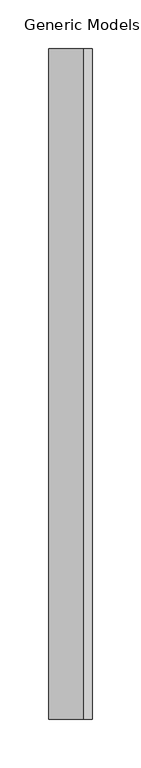
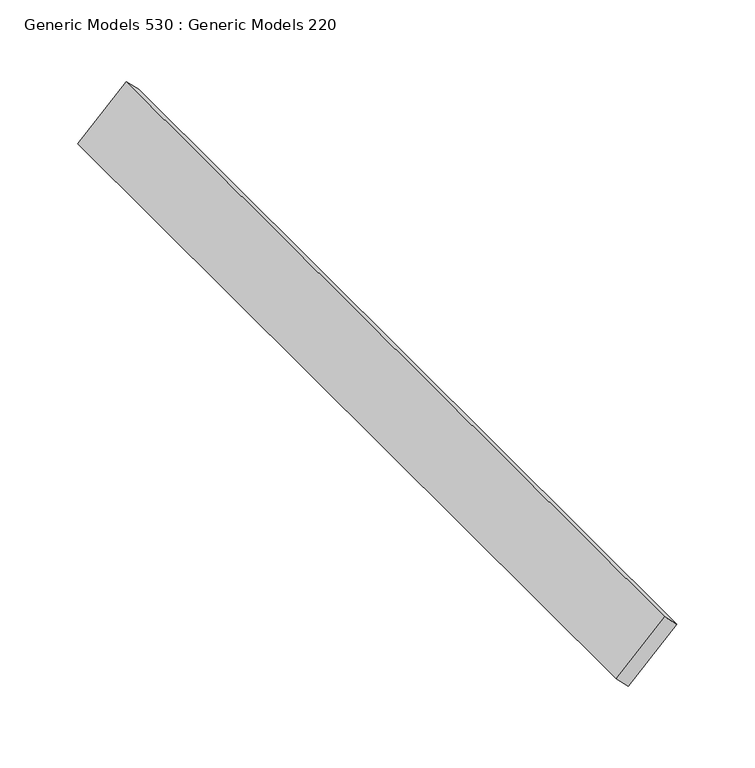
"""IFC4 building model written with IfcOpenShell, lengths in millimetres: proxy geometry, Generic Models 530 : Generic Models 220."""

from ifc_helpers import new_model, si_unit, frame, origin, place, context, project, spatial, polyline, outline, extrude, source, transform, mapped, element, save


def generic_models_530_generic_models_220_b77ca90a(model_context):
    return source(origin(), model_context, "Body", "SweptSolid", [
        extrude(outline(polyline([(0.0, -12.7000001), (0.0, 0.0), (690.8142348, 0.0), (690.8142348, -12.7000001), (0.0, -12.7000001)])), frame((7841.3059863, 4539.4872686, 125319.1399101), z_axis=(0.7071067811868034, 0.0, 0.7071067811862918), x_axis=(0.0, -1.0, 0.0)), (0.0, 0.0, 1.0), 50.8),
    ])


if __name__ == "__main__":
    model = new_model("IFC4")
    model_context = context("Model", 3, world=origin())
    ifc_project = project(units=[si_unit("LENGTHUNIT", "METRE", prefix="MILLI")], contexts=[model_context])
    site = spatial("IfcSite", under=ifc_project)
    building = spatial("IfcBuilding", under=site)
    placement = place(None, origin())
    generic_models_530_generic_models_220_shape = generic_models_530_generic_models_220_b77ca90a(model_context)
    element("IfcBuildingElementProxy", 1, Name="Generic Models 530 : Generic Models 220", ObjectType="Generic Models 530 : Generic Models 220", at=placement, inside=building, context=model_context, shape_type="MappedRepresentation", body=[
        mapped(generic_models_530_generic_models_220_shape, transform((0.0, 0.0, 0.0), x_axis=(1.0, 0.0, 0.0), y_axis=(0.0, 1.0, 0.0), z_axis=(0.0, 0.0, 1.0))),
    ])
    save(model, "model.ifc")

# Revit data of these elements
# Element 1 (IfcBuildingElementProxy, "Generic Models 530 : Generic Models 220")
#   Materials on its faces: "_WOOD TONE ALUMINUM EXTRUSION SLAT BY KNOTWOOD"
# Materials
#   "_WOOD TONE ALUMINUM EXTRUSION SLAT BY KNOTWOOD": class "Generic", colour RGB 177 130 114, transparency 0, Cost = 0
